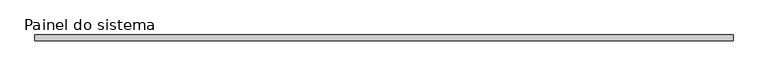
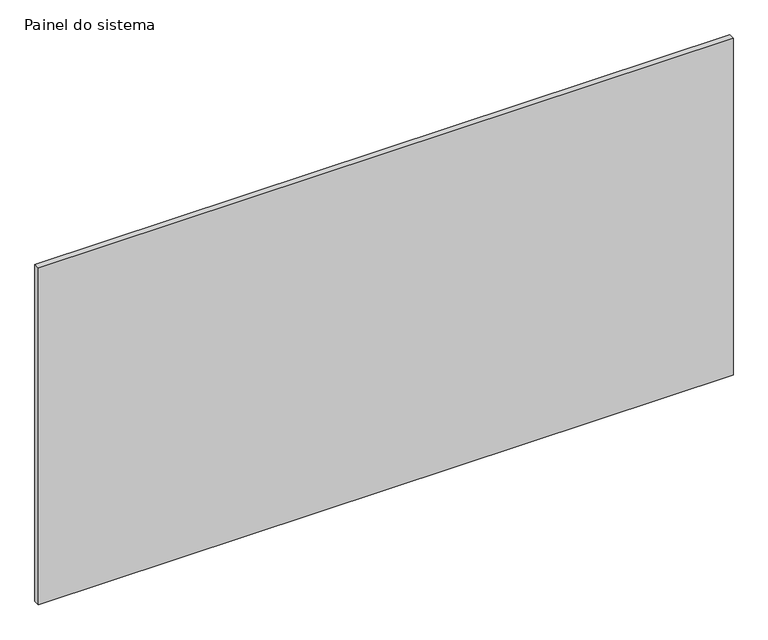
"""IFC4 building model written with IfcOpenShell, lengths in millimetres: plate geometry, Painel do sistema : Envidraçado."""

from ifc_helpers import new_model, si_unit, origin, origin_with_axes, place, context, project, spatial, polyline, outline, extrude, source, transform, mapped, element, save


def painel_do_sistema_9c2734b9(model_context):
    return source(origin(), model_context, "Body", "SweptSolid", [
        extrude(outline(polyline([(1462.5000336, -49.5), (-1462.5000336, -49.5), (-1462.5000336, -24.5), (1462.5000336, -24.5), (1462.5000336, -49.5)])), origin_with_axes(), (0.0, 0.0, 1.0), 1500.0),
    ])


if __name__ == "__main__":
    model = new_model("IFC4")
    model_context = context("Model", 3, world=origin())
    ifc_project = project(units=[si_unit("LENGTHUNIT", "METRE", prefix="MILLI")], contexts=[model_context])
    site = spatial("IfcSite", under=ifc_project)
    building = spatial("IfcBuilding", under=site)
    placement = place(None, origin())
    painel_do_sistema_shape = painel_do_sistema_9c2734b9(model_context)
    element("IfcPlate", 1, ObjectType="Painel do sistema : Envidraçado", at=placement, inside=building, context=model_context, shape_type="MappedRepresentation", body=[
        mapped(painel_do_sistema_shape, transform((0.0, 0.0, 0.0), x_axis=(1.0, 0.0, 0.0), y_axis=(0.0, 1.0, 0.0), z_axis=(0.0, 0.0, 1.0))),
    ])
    save(model, "model.ifc")

# Revit data of these elements
# Type "Painel do sistema : Envidraçado"
#   Construction Type Id = "GSP4R"
#   Analytic Construction = "Vidraça única Pilkington 1/8 pol"
#   Visual Light Transmittance = 0.9
#   Solar Heat Gain Coefficient = 0.86
#   Heat Transfer Coefficient (U) = 6.7069 W/(m²·K)
# Element 1 (IfcPlate, "Painel do sistema : Envidraçado")
#   Materials on its faces: "Vidro"
# Materials
#   "Vidro": class "Vidro", colour RGB 0 128 192, transparency 0.9, Description = "Vidro de sílica", Cost = 0
